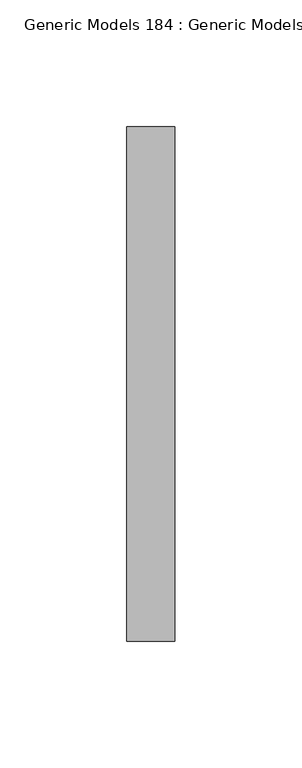
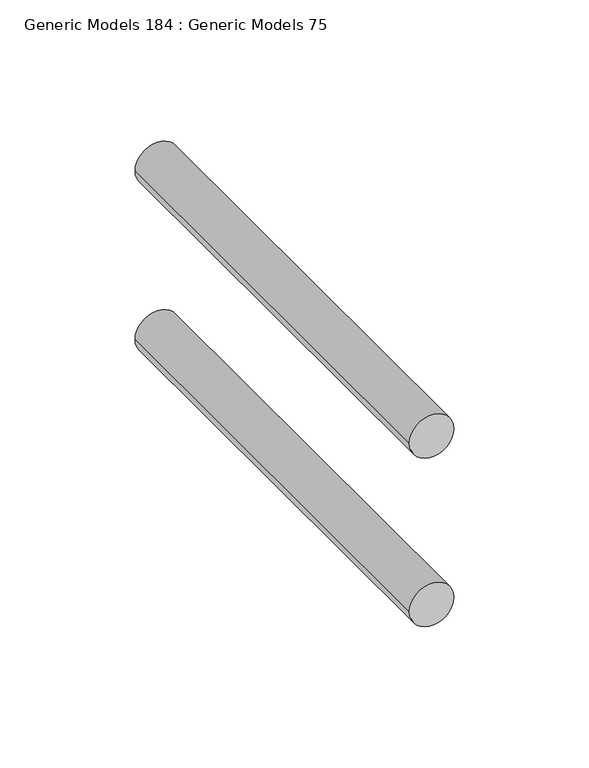
"""IFC4 building model written with IfcOpenShell, lengths in millimetres: proxy geometry, Generic Models 184 : Generic Models 75."""

from ifc_helpers import new_model, si_unit, point, frame, frame_2d, origin, place, context, project, spatial, circle_curve, trimmed, segment, composite_curve, outline, extrude, source, transform, mapped, element, save


def generic_models_184_generic_models_75_7097d878(model_context):
    return source(origin(), model_context, "Body", "SweptSolid", [
        extrude(outline(composite_curve([segment(trimmed(circle_curve(frame_2d((271267.2375, 31975.4096032)), 9.525), [point((271267.2375, 31965.8846032))], [point((271267.2375, 31984.9346032))], False, "CARTESIAN"), True, "CONTINUOUS"), segment(trimmed(circle_curve(frame_2d((271267.2375, 31975.4096032)), 9.525), [point((271267.2375, 31984.9346032))], [point((271267.2375, 31965.8846032))], False, "CARTESIAN"), True, "CONTINUOUS")], self_intersect=False)), frame((0.0, 36305.8207942, 0.0), z_axis=(0.0, 1.0, 0.0), x_axis=(0.0, 0.0, 1.0)), (0.0, 0.0, 1.0), 203.2),
        extrude(outline(composite_curve([segment(trimmed(circle_curve(frame_2d((271343.4375, 31975.4096032)), 9.525), [point((271343.4375, 31965.8846032))], [point((271343.4375, 31984.9346032))], False, "CARTESIAN"), True, "CONTINUOUS"), segment(trimmed(circle_curve(frame_2d((271343.4375, 31975.4096032)), 9.525), [point((271343.4375, 31984.9346032))], [point((271343.4375, 31965.8846032))], False, "CARTESIAN"), True, "CONTINUOUS")], self_intersect=False)), frame((0.0, 36305.8207942, 0.0), z_axis=(0.0, 1.0, 0.0), x_axis=(0.0, 0.0, 1.0)), (0.0, 0.0, 1.0), 203.2),
    ])


if __name__ == "__main__":
    model = new_model("IFC4")
    model_context = context("Model", 3, world=origin())
    ifc_project = project(units=[si_unit("LENGTHUNIT", "METRE", prefix="MILLI")], contexts=[model_context])
    site = spatial("IfcSite", under=ifc_project)
    building = spatial("IfcBuilding", under=site)
    placement = place(None, origin())
    generic_models_184_generic_models_75_shape = generic_models_184_generic_models_75_7097d878(model_context)
    element("IfcBuildingElementProxy", 1, Name="Generic Models 184 : Generic Models 75", ObjectType="Generic Models 184 : Generic Models 75", at=placement, inside=building, context=model_context, shape_type="MappedRepresentation", body=[
        mapped(generic_models_184_generic_models_75_shape, transform((0.0, 0.0, 0.0), x_axis=(1.0, 0.0, 0.0), y_axis=(0.0, 1.0, 0.0), z_axis=(0.0, 0.0, 1.0))),
    ])
    save(model, "model.ifc")
